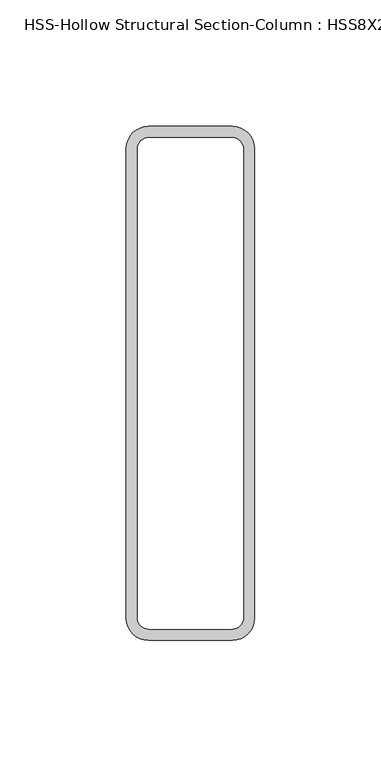
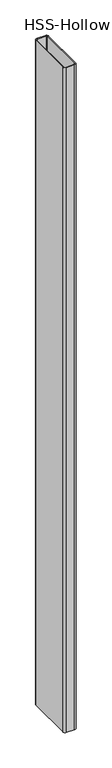
"""IFC4 building model written with IfcOpenShell, lengths in millimetres: column geometry, HSS-Hollow Structural Section-Column : HSS8X2X3/16."""

from ifc_helpers import new_model, si_unit, point, frame, frame_2d, origin, place, context, project, spatial, polyline, circle_curve, trimmed, segment, composite_curve, outline, extrude, source, transform, mapped, element, save


def hss_hollow_structural_section_column_hss8x2x3_16_e82f30fd(model_context):
    return source(origin(), model_context, "Body", "SweptSolid", [
        extrude(outline(composite_curve([segment(trimmed(circle_curve(frame_2d((16.5608, 92.7608)), 8.8392), [point((16.5608, 101.6))], [point((25.4, 92.7608))], False, "CARTESIAN"), True, "CONTINUOUS"), segment(polyline([(25.4, 92.7608), (25.4, -92.7608)]), True, "CONTINUOUS"), segment(trimmed(circle_curve(frame_2d((16.5608, -92.7608)), 8.8392), [point((25.4, -92.7608))], [point((16.5608, -101.6))], False, "CARTESIAN"), True, "CONTINUOUS"), segment(polyline([(16.5608, -101.6), (-16.5608, -101.6)]), True, "CONTINUOUS"), segment(trimmed(circle_curve(frame_2d((-16.5608, -92.7608)), 8.8392), [point((-16.5608, -101.6))], [point((-25.4, -92.7608))], False, "CARTESIAN"), True, "CONTINUOUS"), segment(polyline([(-25.4, -92.7608), (-25.4, 92.7608)]), True, "CONTINUOUS"), segment(trimmed(circle_curve(frame_2d((-16.5608, 92.7608)), 8.8392), [point((-25.4, 92.7608))], [point((-16.5608, 101.6))], False, "CARTESIAN"), True, "CONTINUOUS"), segment(polyline([(-16.5608, 101.6), (16.5608, 101.6)]), True, "CONTINUOUS")], self_intersect=False), holes=[composite_curve([segment(polyline([(16.5608, 97.1804), (-16.5608, 97.1804)]), True, "CONTINUOUS"), segment(trimmed(circle_curve(frame_2d((-16.5608, 92.7608)), 4.4196), [point((-16.5608, 97.1804))], [point((-20.9804, 92.7608))], True, "CARTESIAN"), True, "CONTINUOUS"), segment(polyline([(-20.9804, 92.7608), (-20.9804, -92.7608)]), True, "CONTINUOUS"), segment(trimmed(circle_curve(frame_2d((-16.5608, -92.7608)), 4.4196), [point((-20.9804, -92.7608))], [point((-16.5608, -97.1804))], True, "CARTESIAN"), True, "CONTINUOUS"), segment(polyline([(-16.5608, -97.1804), (16.5608, -97.1804)]), True, "CONTINUOUS"), segment(trimmed(circle_curve(frame_2d((16.5608, -92.7608)), 4.4196), [point((16.5608, -97.1804))], [point((20.9804, -92.7608))], True, "CARTESIAN"), True, "CONTINUOUS"), segment(polyline([(20.9804, -92.7608), (20.9804, 92.7608)]), True, "CONTINUOUS"), segment(trimmed(circle_curve(frame_2d((16.5608, 92.7608)), 4.4196), [point((20.9804, 92.7608))], [point((16.5608, 97.1804))], True, "CARTESIAN"), True, "CONTINUOUS")], self_intersect=False)]), frame((0.0, 0.0, -594.0), z_axis=(0.0, 0.0, 1.0), x_axis=(1.0, 0.0, 0.0)), (0.0, 0.0, 1.0), 2793.0),
    ])


if __name__ == "__main__":
    model = new_model("IFC4")
    model_context = context("Model", 3, world=origin())
    ifc_project = project(units=[si_unit("LENGTHUNIT", "METRE", prefix="MILLI")], contexts=[model_context])
    site = spatial("IfcSite", under=ifc_project)
    building = spatial("IfcBuilding", under=site)
    placement = place(None, origin())
    hss_hollow_structural_section_column_hss8x2x3_16_shape = hss_hollow_structural_section_column_hss8x2x3_16_e82f30fd(model_context)
    element("IfcColumn", 1, ObjectType="HSS-Hollow Structural Section-Column : HSS8X2X3/16", at=placement, inside=building, context=model_context, shape_type="MappedRepresentation", body=[
        mapped(hss_hollow_structural_section_column_hss8x2x3_16_shape, transform((0.0, 0.0, 0.0), x_axis=(1.0, 0.0, 0.0), y_axis=(0.0, 1.0, 0.0), z_axis=(0.0, 0.0, 1.0))),
    ])
    save(model, "model.ifc")

# Revit data of these elements
# Type "HSS-Hollow Structural Section-Column : HSS8X2X3/16"
#   Assembly Code = "B10"
#   Shape = "Rect."
#   Cost = 1
#   W = 12
#   Ht = 203.2 mm
#   b = 50.8 mm
#   kr = 8.839 mm
#   t = 4.42 mm
#   A = 0.00211612 m²
#   Structural Material [instance default] = Steel ASTM A500, Grade B, Rectangular and Square
# Element 1 (IfcColumn, "HSS-Hollow Structural Section-Column : HSS8X2X3/16")
#   Structural Material = Metal - Steel 43-275
#   Materials on its faces: "Metal - Steel 43-275"
# Materials
#   "Steel ASTM A500, Grade B, Rectangular and Square": class "Metal", colour RGB 199 199 199, transparency 0, Description = "Carbon steel", Cost = 0
#   "Metal - Steel 43-275": class "Metal", colour RGB 247 247 247, transparency 0, Cost = 0
